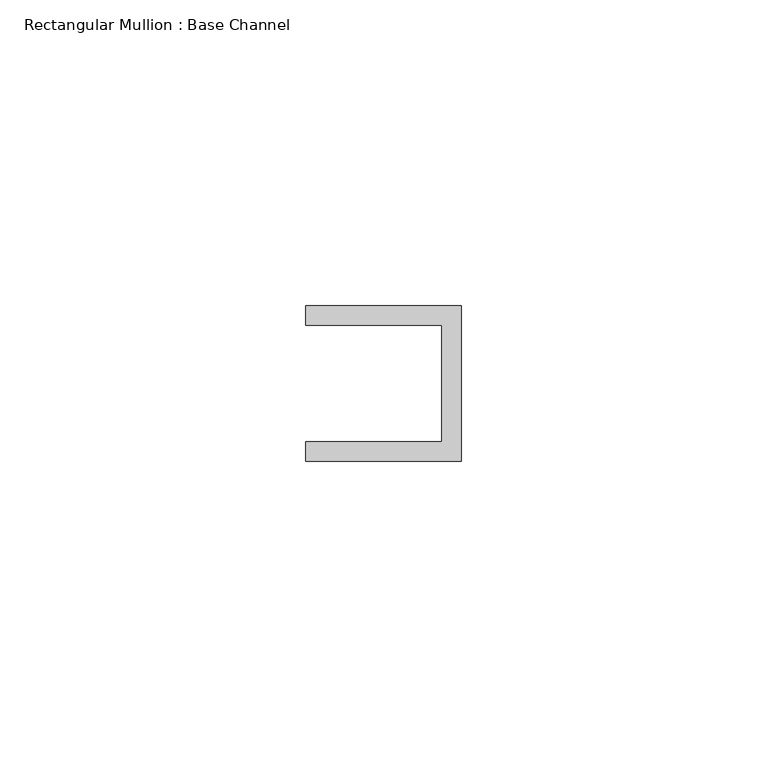
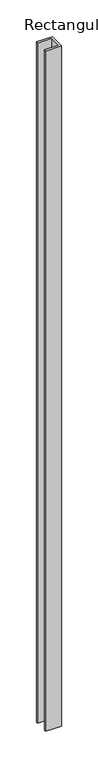
"""IFC4 building model written with IfcOpenShell, lengths in millimetres: member geometry, Rectangular Mullion : Base Channel."""

from ifc_helpers import new_model, si_unit, frame, origin, place, context, project, spatial, polyline, outline, extrude, source, transform, mapped, element, save


def rectangular_mullion_base_channel_ec46be53(model_context):
    return source(origin(), model_context, "Body", "SweptSolid", [
        extrude(outline(polyline([(0.0, 12.7), (0.0, -12.7), (-25.4, -12.7), (-25.4, -9.525), (-3.175, -9.525), (-3.175, 9.525), (-25.4, 9.525), (-25.4, 12.7), (0.0, 12.7)])), frame((0.0, 0.0, -1136.65), z_axis=(0.0, 0.0, 1.0), x_axis=(1.0, 0.0, 0.0)), (0.0, 0.0, 1.0), 1136.65),
    ])


if __name__ == "__main__":
    model = new_model("IFC4")
    model_context = context("Model", 3, world=origin())
    ifc_project = project(units=[si_unit("LENGTHUNIT", "METRE", prefix="MILLI")], contexts=[model_context])
    site = spatial("IfcSite", under=ifc_project)
    building = spatial("IfcBuilding", under=site)
    placement = place(None, origin())
    rectangular_mullion_base_channel_shape = rectangular_mullion_base_channel_ec46be53(model_context)
    element("IfcMember", 1, ObjectType="Rectangular Mullion : Base Channel", at=placement, inside=building, context=model_context, shape_type="MappedRepresentation", body=[
        mapped(rectangular_mullion_base_channel_shape, transform((0.0, 0.0, 0.0), x_axis=(1.0, 0.0, 0.0), y_axis=(0.0, 1.0, 0.0), z_axis=(0.0, 0.0, 1.0))),
    ])
    save(model, "model.ifc")

# Revit data of these elements
# Type "Rectangular Mullion : Base Channel"
#   built-in parameter 1007322 = 0.0833333 (stored number, unit not read)
#   built-in parameter 1007321 = 0.0416667 (stored number, unit not read)
#   built-in parameter 1007320 = -0.03125 (stored number, unit not read)
# Element 1 (IfcMember, "Rectangular Mullion : Base Channel")
#   Materials on its faces: "ALUM"
# Materials
#   "ALUM": class "Generic", colour RGB 157 157 157, transparency 0, Cost = 0
